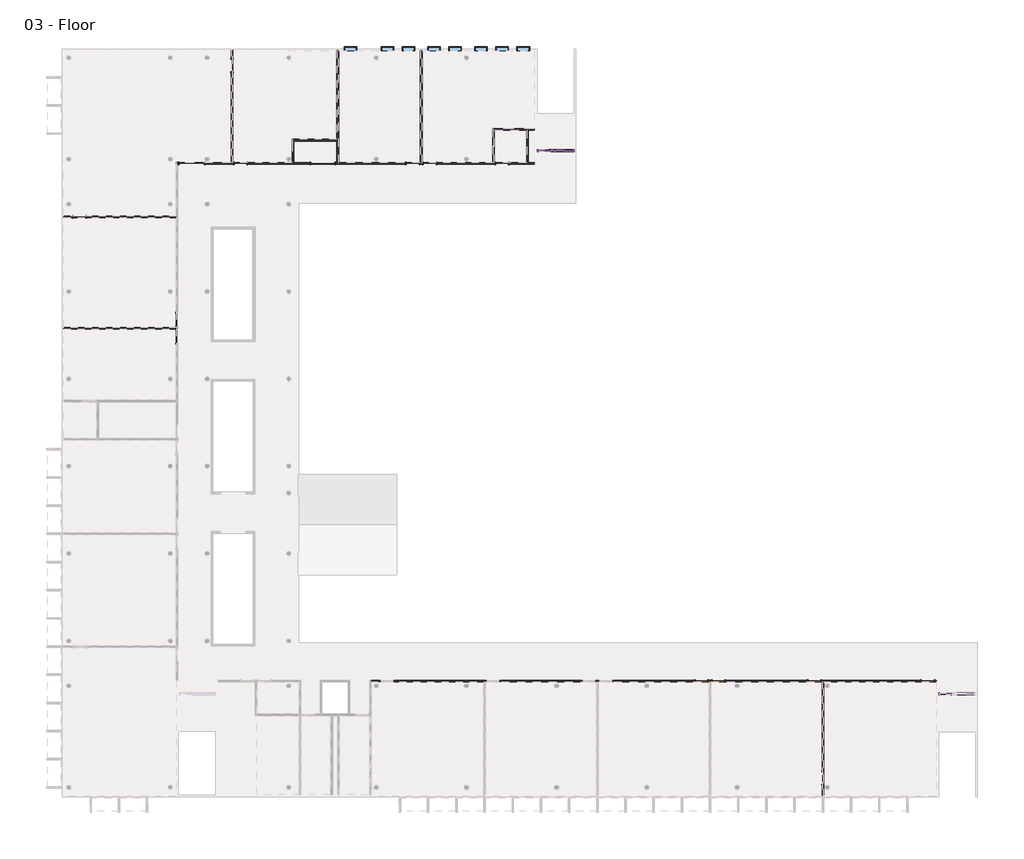
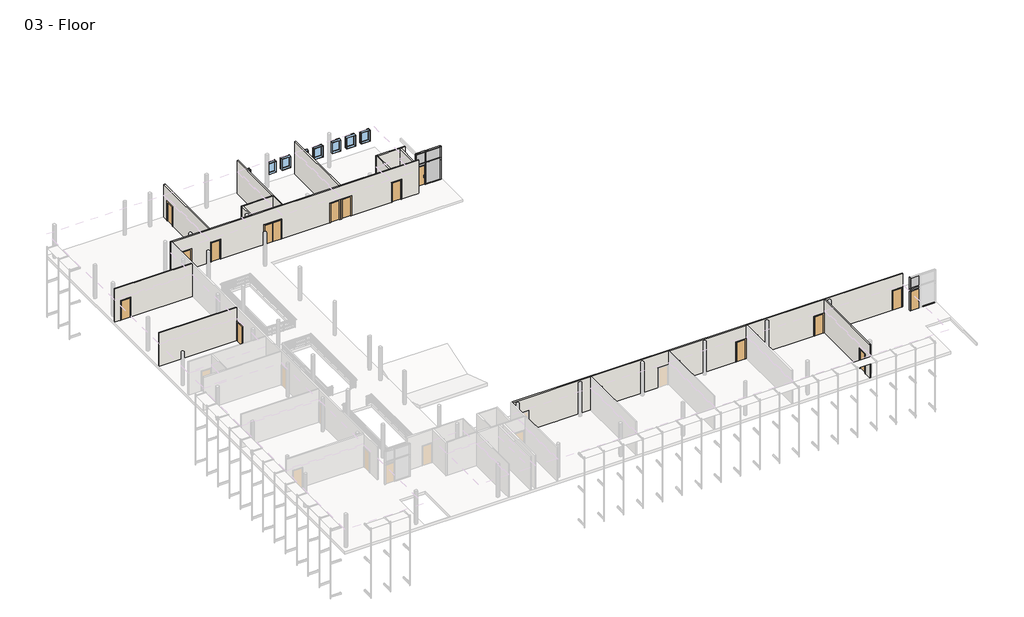
# One storey, part 2 of 4: 22 members, 17 doors, 13 walls, 8 windows, 6 plates.
# Revit data of these elements (continued)
# Type "Curtain Wall Sgl Glass : Curtain Wall Sgl Glass"
#   Assembly Code = "B2030100"
#   Offset = 0' - 2"
#   Function = 1
#   Handle Material = Metal - Aluminum
#   Glazing Material = Glass
# Type "Double-Flush : 68\" x 84\""
#   Type Mark = "10"
#   Assembly Code = "C1020"
#   Thickness = 0' - 2"
#   Height = 7' - 0"
#   Trim Projection Ext = 0' - 1"
#   Trim Projection Int = 0' - 1"
#   Trim Width = 0' - 3"
#   Width = 5' - 8"
#   Function = 0
#   Door Material = Door - Panel
#   Frame Material = Door - Frame
#   Wall Closure = (empty or 0)
# Type "Double-Flush : 72\" x 84\""
#   Type Mark = "12"
#   Assembly Code = "C1020"
#   Thickness = 0' - 2"
#   Height = 7' - 0"
#   Trim Projection Ext = 0' - 1"
#   Trim Projection Int = 0' - 1"
#   Trim Width = 0' - 3"
#   Width = 6' - 0"
#   Function = 0
#   Door Material = Door - Panel
#   Frame Material = Door - Frame
#   Wall Closure = (empty or 0)
# Type "Single-Flush : 36\" x 84\""
#   Type Mark = "1"
#   Assembly Code = "C1020"
#   Thickness = 0' - 2"
#   Height = 7' - 0"
#   Trim Projection Ext = 0' - 1"
#   Trim Projection Int = 0' - 1"
#   Trim Width = 0' - 3"
#   Width = 3' - 0"
#   Function = 0
#   Door Material = Door - Panel
#   Frame Material = Door - Frame
#   Wall Closure = (empty or 0)
# Type "Rectangular Mullion : 2.5\" x 5\" rectangular"
#   built-in parameter 1007304 = 0.416667 (stored number, unit not read)
#   built-in parameter 1007301 = 0.104167 (stored number, unit not read)
#   built-in parameter 1007300 = 0.104167 (stored number, unit not read)
# Type "Typ. Partition Wall"
#   Assembly Code = "B2010"
#   Type Mark = "A1"
#   Width = 0' - 4 1/2"
#   Layers, outside or top first: 0' - 0 1/2" "Gypsum Wall Board" (function 1); 0' - 3 1/2" "Metal - Stud Layer" (function 1); 0' - 0 1/2" "Gypsum Wall Board" (function 1)
# Type "Fixed : 36\" x 48\""
#   Type Mark = "1"
#   Assembly Code = "B2020100"
#   Height = 4' - 0"
#   Default Sill Height = 3' - 0"
#   Width = 3' - 0"
#   Window Inset = 0' - 0 3/4"
#   Glass Pane Material = Glass
#   Sash Material = Sash
#   Wall Closure = (empty or 0)
# Element 1 (IfcDoor, "Curtain Wall Sgl Glass : Curtain Wall Sgl Glass")
#   Frame Material = "Alum."
#   Frame Type = "1"
#   Mark = "327"
#   Phase Created = New Construction
#   Materials on its faces: "Metal - Aluminum", "Glass"
# Element 2 (IfcDoor, "Curtain Wall Sgl Glass : Curtain Wall Sgl Glass")
#   Frame Material = "Alum."
#   Frame Type = "1"
#   Mark = "301"
#   Phase Created = New Construction
#   Materials on its faces: "Metal - Aluminum", "Glass"
# Element 3 (IfcDoor, "Double-Flush : 68\" x 84\"")
#   Frame Material = "Wood"
#   Frame Type = "3"
#   Phase Created = New Construction
#   Materials on its faces: "Door - Frame", "Door - Panel"
# Element 4 (IfcDoor, "Double-Flush : 72\" x 84\"")
#   Frame Material = "Wood"
#   Frame Type = "3"
#   Phase Created = New Construction
#   Materials on its faces: "Door - Frame", "Door - Panel"
# Elements 5, 6, 7, 8, 9, 10, 11, 12, 13, 14, 15, 16, 17 (IfcDoor, "Single-Flush : 36\" x 84\"")
#   Frame Material = "Wood"
#   Frame Type = "3"
#   Phase Created = New Construction
#   Materials on its faces: "Door - Frame", "Door - Panel"
# Elements 18, 19, 20, 21, 22, 23, 24, 25, 26, 27, 28, 29, 30, 31, 32, 33, 34, 35, 36, 37, 38, 39 (IfcMember, "Rectangular Mullion : 2.5\" x 5\" rectangular")
#   Phase Created = New Construction
#   Materials on its faces: "Metal - Aluminum"
# Elements 40, 41, 42, 43, 44, 45 (IfcPlate, "System Panel : Glazed")
#   Phase Created = New Construction
#   Materials on its faces: "Glass"
# Elements 46, 47, 48, 49, 50, 51, 52, 53, 55, 57, 58 (IfcWall, "Typ. Partition Wall")
#   Top Offset = 0' - 0"
#   Base Offset = 0' - 0"
#   wall height = 12' - 0"
#   Phase Created = New Construction
#   Base Constraint = 03 - Floor
#   Top Constraint = Roof
#   Materials on its faces: "Default Wall", "Gypsum Wall Board"
# Elements 54, 56 (IfcWall, "Typ. Partition Wall")
#   Top Offset = 0' - 0"
#   Base Offset = 0' - 0"
#   wall height = 12' - 0"
#   Phase Created = New Construction
#   Base Constraint = 03 - Floor
#   Top Constraint = Roof
#   Materials on its faces: "Gypsum Wall Board", "Default Wall"
# Element 59 (IfcWindow, "Fixed : 36\" x 48\"")
#   Mark = "21"
#   Phase Created = New Construction
#   Materials on its faces: "Sash", "Glass"
# Element 60 (IfcWindow, "Fixed : 36\" x 48\"")
#   Mark = "22"
#   Phase Created = New Construction
#   Materials on its faces: "Sash", "Glass"
# Element 61 (IfcWindow, "Fixed : 36\" x 48\"")
#   Mark = "23"
#   Phase Created = New Construction
#   Materials on its faces: "Sash", "Glass"
# Element 62 (IfcWindow, "Fixed : 36\" x 48\"")
#   Mark = "24"
#   Phase Created = New Construction
#   Materials on its faces: "Sash", "Glass"
# Element 63 (IfcWindow, "Fixed : 36\" x 48\"")
#   Mark = "25"
#   Phase Created = New Construction
#   Materials on its faces: "Sash", "Glass"
# Element 64 (IfcWindow, "Fixed : 36\" x 48\"")
#   Mark = "26"
#   Phase Created = New Construction
#   Materials on its faces: "Sash", "Glass"
# Element 65 (IfcWindow, "Fixed : 36\" x 48\"")
#   Mark = "27"
#   Phase Created = New Construction
#   Materials on its faces: "Sash", "Glass"
# Element 66 (IfcWindow, "Fixed : 36\" x 48\"")
#   Mark = "28"
#   Phase Created = New Construction
#   Materials on its faces: "Sash", "Glass"
# Materials
#   "Metal - Aluminum": class "Metal", colour RGB 140 140 140, transparency 0
#   "Glass": class "Glass", colour RGB 0 128 192, transparency 0.75
#   "Door - Panel": class "Wood", colour RGB 210 159 95, transparency 0
#   "Door - Frame": class "Miscellaneous", colour RGB 118 70 51, transparency 0
#   "Gypsum Wall Board": class "Paint", colour RGB 153 153 153, transparency 0, Description = "Interior finish"
#   "Metal - Stud Layer": class "Metal", colour RGB 199 199 199, transparency 0
#   "Sash": class "Wood", colour RGB 224 178 126, transparency 0
#   "Default Wall": class "Miscellaneous", colour RGB 128 128 128, transparency 0
